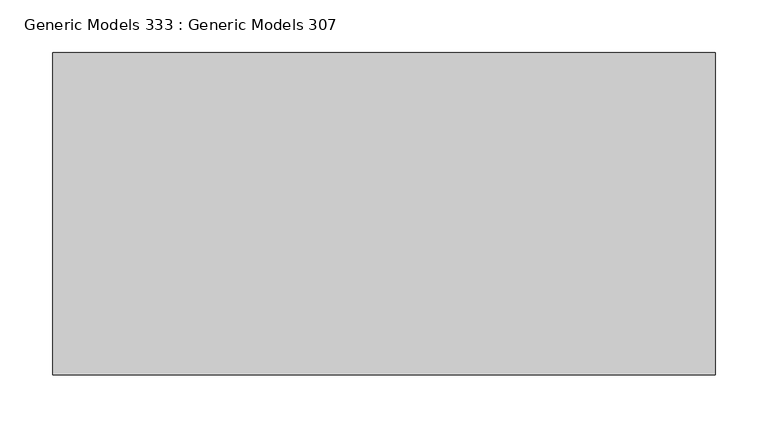
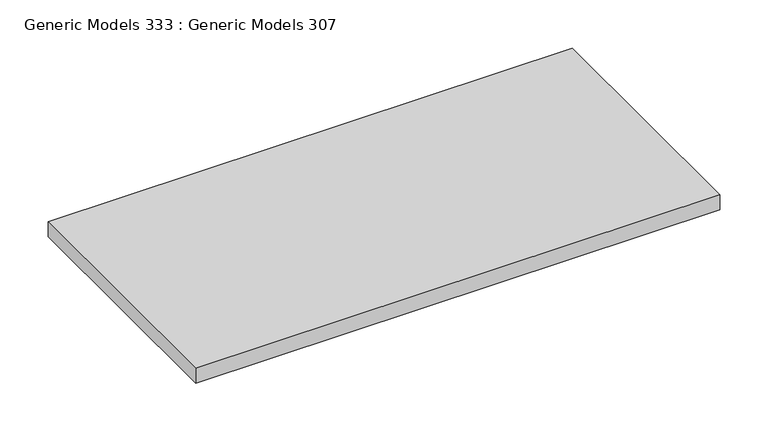
"""IFC4 building model written with IfcOpenShell, lengths in millimetres: proxy geometry, Generic Models 333 : Generic Models 307."""

import ifcopenshell
import ifcopenshell.guid

model = None  # the IFC model being written
_history = None  # IfcOwnerHistory: only IFC2X3 demands one
_inside = {}  # id of a spatial element -> (the spatial element, [elements in it])
_under = {}  # id of a project, library or spatial element -> (it, [spatial elements below it])
_declared = {}  # id of a project -> (the project, [libraries it declares])
_typed = {}  # id of a type object -> (the type object, [elements of that type])
_made_of = {}  # id of a material, layer set ... -> (it, [elements and type objects made of it])


def new_model(schema):
    """Start an empty IFC model of exactly this schema.

    Asked for "IFC4X3", IfcOpenShell would pick the latest addendum, in which some entities
    have other attributes; the version numbers below select the first issue.
    IFC2X3 requires an IfcOwnerHistory on every rooted entity: one is made here for all.
    """
    global model, _history
    if schema == "IFC4X3":
        model = ifcopenshell.file(schema_version=(4, 3, 0, 0))
    else:
        model = ifcopenshell.file(schema=schema)
    _inside.clear()
    _under.clear()
    _declared.clear()
    _typed.clear()
    _made_of.clear()
    _history = None
    if model.schema == "IFC2X3":
        org = make("IfcOrganization", Name="unknown")
        user = make(
            "IfcPersonAndOrganization",
            ThePerson=make("IfcPerson", FamilyName="unknown"),
            TheOrganization=org,
        )
        app = make(
            "IfcApplication",
            ApplicationDeveloper=org,
            Version="unknown",
            ApplicationFullName="unknown",
            ApplicationIdentifier="unknown",
        )
        _history = make(
            "IfcOwnerHistory",
            OwningUser=user,
            OwningApplication=app,
            ChangeAction="ADDED",
            CreationDate=0,
        )
    return model


def make(cls, **values):
    """One entity of the class cls with the attributes given. An attribute that is None is left unset."""
    return model.create_entity(
        cls, **{name: value for name, value in values.items() if value is not None}
    )


def rooted(cls, **values):
    """An entity with a GlobalId (a new one), such as an element, a storey or a relation."""
    return make(cls, GlobalId=ifcopenshell.guid.new(), OwnerHistory=_history, **values)


def si_unit(unit_type, name, prefix=None):
    """IfcSIUnit, for example si_unit("LENGTHUNIT", "METRE", prefix="MILLI")."""
    return make("IfcSIUnit", UnitType=unit_type, Prefix=prefix, Name=name)


def assignment(units):
    """IfcUnitAssignment: the units of a project."""
    return None if units is None else make("IfcUnitAssignment", Units=units)


def point(xyz):
    """IfcCartesianPoint."""
    return None if xyz is None else make("IfcCartesianPoint", Coordinates=xyz)


def direction(xyz):
    """IfcDirection."""
    return None if xyz is None else make("IfcDirection", DirectionRatios=xyz)


def frame(location, z_axis=None, x_axis=None):
    """IfcAxis2Placement3D, a coordinate frame: its origin and axes. An axis left out is left unset."""
    return make(
        "IfcAxis2Placement3D",
        Location=point(location),
        Axis=direction(z_axis),
        RefDirection=direction(x_axis),
    )


def origin():
    """The frame at (0, 0, 0) with its axes left unset."""
    return frame((0.0, 0.0, 0.0))


def place(relative_to, where):
    """IfcLocalPlacement: puts the frame where relative to a parent placement (None: the world)."""
    return make(
        "IfcLocalPlacement", PlacementRelTo=relative_to, RelativePlacement=where
    )


def context(
    kind, dimensions, precision=None, world=None, true_north=None, identifier=None
):
    """IfcGeometricRepresentationContext, for example the 3D "Model" context."""
    return make(
        "IfcGeometricRepresentationContext",
        ContextIdentifier=identifier,
        ContextType=kind,
        CoordinateSpaceDimension=dimensions,
        Precision=precision,
        WorldCoordinateSystem=world,
        TrueNorth=true_north,
    )


def project(units=None, contexts=None):
    """IfcProject with its units and contexts."""
    return rooted(
        "IfcProject",
        Name="project",
        RepresentationContexts=contexts,
        UnitsInContext=assignment(units),
    )


def spatial(cls, under=None, at=None, **own):
    """A site, building, storey or space (cls), placed at a placement, below another one or the project."""
    s = rooted(cls, ObjectPlacement=at, **own)
    if under is not None:
        _under.setdefault(under.id(), (under, []))[1].append(s)
    return s


def polyline(points):
    """IfcPolyline through the points."""
    return make("IfcPolyline", Points=[point(p) for p in points])


def outline(outer, holes=None, kind="AREA"):
    """IfcArbitraryClosedProfileDef: a profile drawn as a closed curve; with holes, ...WithVoids."""
    if holes is None:
        return make("IfcArbitraryClosedProfileDef", ProfileType=kind, OuterCurve=outer)
    return make(
        "IfcArbitraryProfileDefWithVoids",
        ProfileType=kind,
        OuterCurve=outer,
        InnerCurves=holes,
    )


def extrude(swept, where, along, depth):
    """IfcExtrudedAreaSolid: the profile swept, set in the frame where, extruded along a direction by depth."""
    return make(
        "IfcExtrudedAreaSolid",
        SweptArea=swept,
        Position=where,
        ExtrudedDirection=direction(along),
        Depth=depth,
    )


def shape(context_of_items, identifier, shape_type, items):
    """IfcShapeRepresentation: the items that make up one representation, for example the "Body"."""
    return make(
        "IfcShapeRepresentation",
        ContextOfItems=context_of_items,
        RepresentationIdentifier=identifier,
        RepresentationType=shape_type,
        Items=items,
    )


def source(mapping_origin, context_of_items, identifier, shape_type, items):
    """IfcRepresentationMap: a shape defined once, which mapped items show again and again."""
    return make(
        "IfcRepresentationMap",
        MappingOrigin=mapping_origin,
        MappedRepresentation=shape(context_of_items, identifier, shape_type, items),
    )


def transform(
    local_origin,
    x_axis=None,
    y_axis=None,
    z_axis=None,
    scale=None,
    scale2=None,
    scale3=None,
    uniform=True,
):
    """IfcCartesianTransformationOperator3D, or its non-uniform kind. x_axis, y_axis, z_axis: its Axis1, 2, 3."""
    if uniform:
        return make(
            "IfcCartesianTransformationOperator3D",
            Axis1=direction(x_axis),
            Axis2=direction(y_axis),
            LocalOrigin=point(local_origin),
            Scale=scale,
            Axis3=direction(z_axis),
        )
    return make(
        "IfcCartesianTransformationOperator3DnonUniform",
        Axis1=direction(x_axis),
        Axis2=direction(y_axis),
        LocalOrigin=point(local_origin),
        Scale=scale,
        Axis3=direction(z_axis),
        Scale2=scale2,
        Scale3=scale3,
    )


def mapped(mapping_source, mapping_target):
    """IfcMappedItem: shows the shape of a source again, moved by a transform."""
    return make(
        "IfcMappedItem", MappingSource=mapping_source, MappingTarget=mapping_target
    )


def made_of(thing, what):
    """Note that an element or type object is made of a material, layer set ...; save() writes the relation."""
    if what is not None:
        _made_of.setdefault(what.id(), (what, []))[1].append(thing)
    return thing


def element(
    cls,
    number,
    at=None,
    inside=None,
    cuts=None,
    type_object=None,
    material=None,
    context=None,
    identifier="Body",
    shape_type=None,
    held_by="IfcProductDefinitionShape",
    body=None,
    shapes=None,
    **own,
):
    """One element of the class cls, such as IfcWall. Its Tag is "e" and its number.

    at: its placement. inside: the storey or other place that contains it. cuts: it is an
    opening in that element (IfcRelVoidsElement). A single representation is given by context,
    identifier, shape_type and body (its items); several are given by shapes. held_by: the class
    of the entity that holds the representations. save() writes the other relations.
    """
    e = rooted(cls, Tag="e%d" % number, ObjectPlacement=at, **own)
    if body is not None:
        shapes = [shape(context, identifier, shape_type, body)]
    if shapes is not None:
        e.Representation = make(held_by, Representations=shapes)
    if inside is not None:
        _inside.setdefault(inside.id(), (inside, []))[1].append(e)
    if cuts is not None:
        rooted(
            "IfcRelVoidsElement", RelatingBuildingElement=cuts, RelatedOpeningElement=e
        )
    if type_object is not None:
        _typed.setdefault(type_object.id(), (type_object, []))[1].append(e)
    return made_of(e, material)


def aggregate(whole, parts):
    """IfcRelAggregates: a whole, such as a stair, and the parts it consists of."""
    return rooted("IfcRelAggregates", RelatingObject=whole, RelatedObjects=parts)


def save(model, path):
    """Write the relations noted so far, then the file.

    IfcRelAggregates (storeys below a building ...), IfcRelContainedInSpatialStructure (elements
    in a storey), IfcRelDefinesByType, IfcRelAssociatesMaterial and IfcRelDeclares: one each for
    every whole, place, type object, material and project.
    """
    for whole, parts in _under.values():
        aggregate(whole, parts)
    for where, things in _inside.values():
        rooted(
            "IfcRelContainedInSpatialStructure",
            RelatedElements=things,
            RelatingStructure=where,
        )
    for kind, things in _typed.values():
        rooted("IfcRelDefinesByType", RelatedObjects=things, RelatingType=kind)
    for what, things in _made_of.values():
        rooted("IfcRelAssociatesMaterial", RelatedObjects=things, RelatingMaterial=what)
    for by, libraries in _declared.values():
        rooted("IfcRelDeclares", RelatingContext=by, RelatedDefinitions=libraries)
    model.write(path)


def generic_models_333_generic_models_307_5991fbdf(model_context):
    return source(origin(), model_context, "Body", "SweptSolid", [
        extrude(outline(polyline([(4952.0863544, 704.5309662), (5578.4173784, 704.5309662), (5578.4173784, 399.7309662), (4952.0863544, 399.7309662), (4952.0863544, 704.5309662)])), frame((0.0, 0.0, 129228.596), z_axis=(0.0, 0.0, 1.0), x_axis=(1.0, 0.0, 0.0)), (0.0, 0.0, 1.0), 19.05),
    ])


if __name__ == "__main__":
    model = new_model("IFC4")
    model_context = context("Model", 3, world=origin())
    ifc_project = project(units=[si_unit("LENGTHUNIT", "METRE", prefix="MILLI")], contexts=[model_context])
    site = spatial("IfcSite", under=ifc_project)
    building = spatial("IfcBuilding", under=site)
    placement = place(None, origin())
    generic_models_333_generic_models_307_shape = generic_models_333_generic_models_307_5991fbdf(model_context)
    element("IfcBuildingElementProxy", 1, Name="Generic Models 333 : Generic Models 307", ObjectType="Generic Models 333 : Generic Models 307", at=placement, inside=building, context=model_context, shape_type="MappedRepresentation", body=[
        mapped(generic_models_333_generic_models_307_shape, transform((0.0, 0.0, 0.0), x_axis=(1.0, 0.0, 0.0), y_axis=(0.0, 1.0, 0.0), z_axis=(0.0, 0.0, 1.0))),
    ])
    save(model, "model.ifc")

# Revit data of these elements
# Element 1 (IfcBuildingElementProxy, "Generic Models 333 : Generic Models 307")
#   Materials on its faces: "FIRE RETARDANT TREATED WOOD SOFFIT"
# Materials
#   "FIRE RETARDANT TREATED WOOD SOFFIT": class "Generic", colour RGB 177 130 114, transparency 0, Cost = 0
